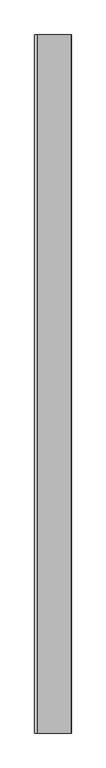
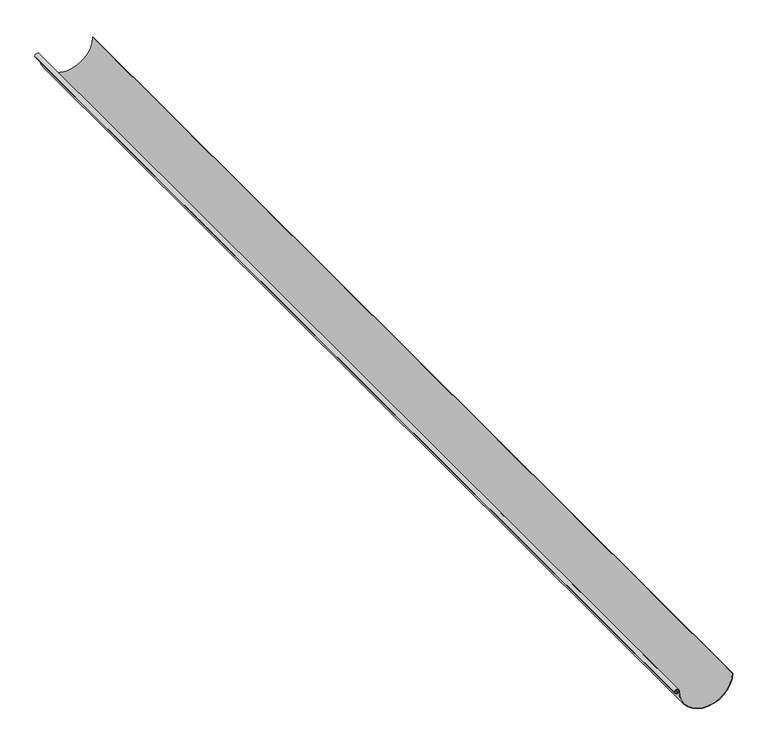
"""IFC4 building model written with IfcOpenShell, lengths in millimetres: proxy geometry, Inner panel:Inner panel:1:Inner panel:1 : Inner panel:Inner panel:300324:2:Inner panel:1:Inner panel:1 : Inner panel:Inner panel:300324:2 : Inner panel:Inner panel:1:Inner panel:1 : Inner panel:Inner panel:300324:300043:30 : Inner panel:Inner panel:1:Inner panel:1 : Inner panel:Inner panel:300324:2:Inner panel:1:Inner panel:1 : Inner panel:Inner panel:300324:2 : Inner panel:Inner panel:1:Inner panel:1 : Inner panel:Inner panel:300324:300043:308120."""

from ifc_helpers import new_model, si_unit, point, frame, frame_2d, origin, place, context, project, spatial, polyline, circle_curve, trimmed, segment, composite_curve, outline, extrude, source, transform, mapped, element, save


def generic_models_6cdf0552(model_context):
    return source(origin(), model_context, "Body", "SweptSolid", [
        extrude(outline(composite_curve([segment(polyline([(3815.4372291, 558129.4037733), (3815.4372291, 558127.8162733)]), True, "CONTINUOUS"), segment(trimmed(circle_curve(frame_2d((3815.4372291, 558040.5037733)), 87.3125), [point((3815.4372291, 558127.8162733))], [point((3815.4372291, 557953.1912733))], True, "CARTESIAN"), True, "CONTINUOUS"), segment(trimmed(circle_curve(frame_2d((3815.4372291, 557945.4213027)), 7.7699706), [point((3815.4372291, 557953.1912733))], [point((3809.3011565, 557950.1879636))], False, "CARTESIAN"), True, "CONTINUOUS"), segment(polyline([(3809.3011565, 557950.1879636), (3810.4348098, 557949.0543103)]), True, "CONTINUOUS"), segment(trimmed(circle_curve(frame_2d((3815.4372291, 557945.4213027)), 6.1824706), [point((3810.4348098, 557949.0543103))], [point((3815.4372291, 557951.6037733))], True, "CARTESIAN"), True, "CONTINUOUS"), segment(trimmed(circle_curve(frame_2d((3815.4372291, 558040.5037733)), 88.9), [point((3815.4372291, 557951.6037733))], [point((3815.4372291, 558129.4037733))], False, "CARTESIAN"), True, "CONTINUOUS")], self_intersect=False)), frame((0.0, -582008.5744985, 0.0), z_axis=(0.0, 1.0, 0.0), x_axis=(0.0, 0.0, 1.0)), (0.0, 0.0, 1.0), 3657.6),
    ])


if __name__ == "__main__":
    model = new_model("IFC4")
    model_context = context("Model", 3, world=origin())
    ifc_project = project(units=[si_unit("LENGTHUNIT", "METRE", prefix="MILLI")], contexts=[model_context])
    site = spatial("IfcSite", under=ifc_project)
    building = spatial("IfcBuilding", under=site)
    placement = place(None, origin())
    generic_models_shape = generic_models_6cdf0552(model_context)
    element("IfcBuildingElementProxy", 1, Name="Inner panel:Inner panel:1:Inner panel:1 : Inner panel:Inner panel:300324:2:Inner panel:1:Inner panel:1 : Inner panel:Inner panel:300324:2 : Inner panel:Inner panel:1:Inner panel:1 : Inner panel:Inner panel:300324:300043:30 : Inner panel:Inner panel:1:Inner panel:1 : Inner panel:Inner panel:300324:2:Inner panel:1:Inner panel:1 : Inner panel:Inner panel:300324:2 : Inner panel:Inner panel:1:Inner panel:1 : Inner panel:Inner panel:300324:300043:308120", ObjectType="Inner panel:Inner panel:1:Inner panel:1 : Inner panel:Inner panel:300324:2:Inner panel:1:Inner panel:1 : Inner panel:Inner panel:300324:2 : Inner panel:Inner panel:1:Inner panel:1 : Inner panel:Inner panel:300324:300043:30 : Inner panel:Inner panel:1:Inner panel:1 : Inner panel:Inner panel:300324:2:Inner panel:1:Inner panel:1 : Inner panel:Inner panel:300324:2 : Inner panel:Inner panel:1:Inner panel:1 : Inner panel:Inner panel:300324:300043:308120", at=placement, inside=building, context=model_context, shape_type="MappedRepresentation", body=[
        mapped(generic_models_shape, transform((0.0, 0.0, 0.0), x_axis=(1.0, 0.0, 0.0), y_axis=(0.0, 1.0, 0.0), z_axis=(0.0, 0.0, 1.0))),
    ])
    save(model, "model.ifc")

# Revit data of these elements
# Type "Inner panel:Inner panel:1:Inner panel:1 : Inner panel:Inner panel:300324:2:Inner panel:1:Inner panel:1 : Inner panel:Inner panel:300324:2 : Inner panel:Inner panel:1:Inner panel:1 : Inner panel:Inner panel:300324:300043:30 : Inner panel:Inner panel:1:Inner panel:1 : Inner panel:Inner panel:300324:2:Inner panel:1:Inner panel:1 : Inner panel:Inner panel:300324:2 : Inner panel:Inner panel:1:Inner panel:1 : Inner panel:Inner panel:300324:300043:308120"
#   NameOverride = "Inner panel:Inner panel:1:Inner panel:1 : Inner panel:Inner panel:300324:2:Inner panel:1:Inner panel:1 : Inner panel:Inner panel:300324:2 : Inner panel:Inner panel:1:Inner panel:1 : Inner panel:Inner panel:300324:300043:308120"
#   ObjectTypeOverride = "Inner panel:1:Inner panel:1 : Inner panel:Inner panel:300324:2 : Inner panel:Inner panel:1:Inner panel:1 : Inner panel:Inner panel:300324:300043"
#   Reference = "Inner panel"
#   Tag = "308120"
# Element 1 (IfcBuildingElementProxy, "Inner panel:Inner panel:1:Inner panel:1 : Inner panel:Inner panel:300324:2:Inner panel:1:Inner panel:1 : Inner panel:Inner panel:300324:2 : Inner panel:Inner panel:1:Inner panel:1 : Inner panel:Inner panel:300324:300043:30 : Inner panel:Inner panel:1:Inner panel:1 : Inner panel:Inner panel:300324:2:Inner panel:1:Inner panel:1 : Inner panel:Inner panel:300324:2 : Inner panel:Inner panel:1:Inner panel:1 : Inner panel:Inner panel:300324:300043:308120")
#   Materials on its faces: "HALF-ROUND GUTTERS"
# Materials
#   "HALF-ROUND GUTTERS": class "Unassigned", colour RGB 210 209 208, transparency 0, Cost = 0
